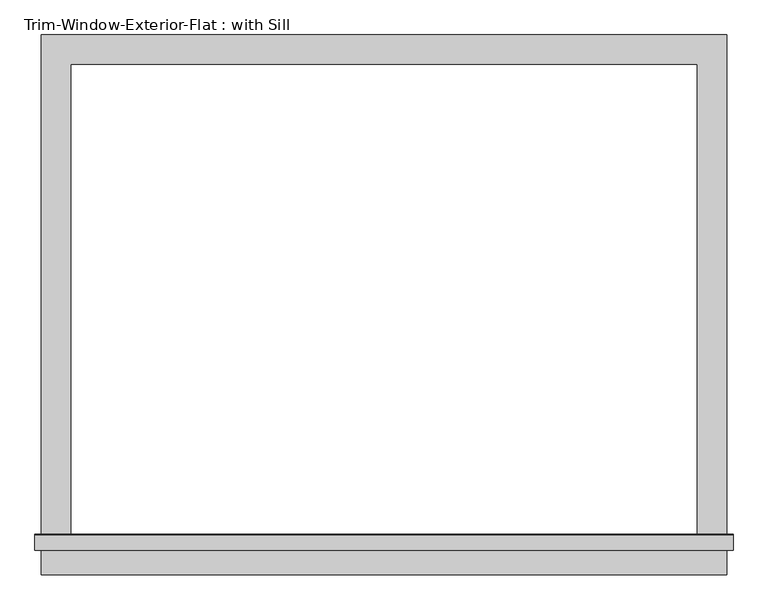
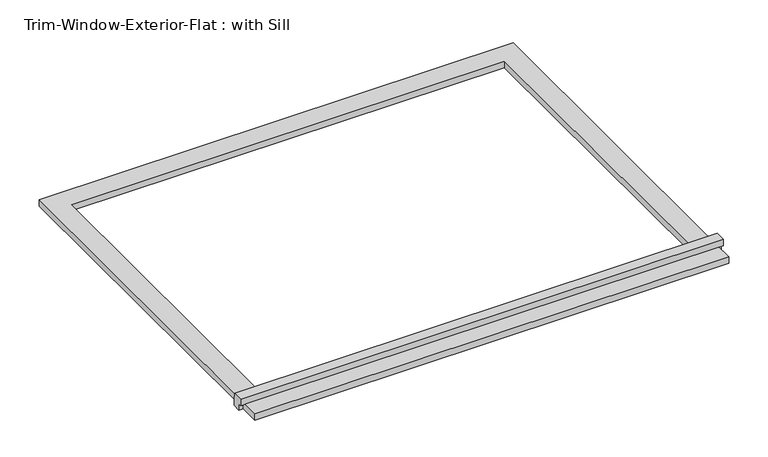
"""IFC4 building model written with IfcOpenShell, lengths in millimetres: proxy geometry, Trim-Window-Exterior-Flat : with Sill."""

from ifc_helpers import new_model, si_unit, frame, origin, origin_with_axes, place, context, project, spatial, polyline, outline, extrude, source, transform, mapped, element, save


def trim_window_exterior_flat_with_sill_c4e67c73(model_context):
    return source(origin(), model_context, "Body", "SweptSolid", [
        extrude(outline(polyline([(666.75, -936.5823709), (666.75, -993.7323709), (-666.75, -993.7323709), (-666.75, -936.5823709), (666.75, -936.5823709)])), origin_with_axes(), (0.0, 0.0, 1.0), 19.05),
        extrude(outline(polyline([(-946.15, 38.1), (-916.8580645, 38.1), (-914.4, 19.05), (-914.4, 0.0), (-936.5823709, 0.0), (-936.5823709, 19.05), (-946.15, 19.05), (-946.15, 38.1)])), frame((-679.45, 0.0, 0.0), z_axis=(1.0, 0.0, 0.0), x_axis=(0.0, 1.0, 0.0)), (0.0, 0.0, 1.0), 1358.9),
        extrude(outline(polyline([(-666.75, 57.15), (666.75, 57.15), (666.75, -914.4), (609.6, -914.4), (609.6, 0.0), (-609.6, 0.0), (-609.6, -914.4), (-666.75, -914.4), (-666.75, 57.15)])), origin_with_axes(), (0.0, 0.0, 1.0), 19.05),
    ])


if __name__ == "__main__":
    model = new_model("IFC4")
    model_context = context("Model", 3, world=origin())
    ifc_project = project(units=[si_unit("LENGTHUNIT", "METRE", prefix="MILLI")], contexts=[model_context])
    site = spatial("IfcSite", under=ifc_project)
    building = spatial("IfcBuilding", under=site)
    placement = place(None, origin())
    trim_window_exterior_flat_with_sill_shape = trim_window_exterior_flat_with_sill_c4e67c73(model_context)
    element("IfcBuildingElementProxy", 1, Name="Trim-Window-Exterior-Flat : with Sill", ObjectType="Trim-Window-Exterior-Flat : with Sill", at=placement, inside=building, context=model_context, shape_type="MappedRepresentation", body=[
        mapped(trim_window_exterior_flat_with_sill_shape, transform((0.0, 0.0, 0.0), x_axis=(1.0, 0.0, 0.0), y_axis=(0.0, 1.0, 0.0), z_axis=(0.0, 0.0, 1.0))),
    ])
    save(model, "model.ifc")

# Revit data of these elements
# Type "Trim-Window-Exterior-Flat : with Sill"
#   Trim Width = 0' - 2 1/4"
#   Trim Thickness_Picture Frame = 0' - 1 1/4"
#   Trim Thickness_with Sill = 0' - 0 3/4"
#   Sill Thickness = 0' - 1 1/4"
#   Opening Width [instance default] = 2' - 0"
#   Opening Height [instance default] = 3' - 0"
#   Default Elevation = 4' - 0"
#   Sill = yes
#   Picture Frame = no
#   Trim Material [instance default] = none
# Element 1 (IfcBuildingElementProxy, "Trim-Window-Exterior-Flat : with Sill")
#   Opening Width = 4' - 0"
#   Trim Material = EXISTING DRYWALL (PAINTED)
#   Materials on its faces: "EXISTING DRYWALL (PAINTED)"
# Materials
#   "EXISTING DRYWALL (PAINTED)": class "Wood", colour RGB 80 80 80, transparency 0, Description = "Wood framing, thermal airspace", Cost = 0
